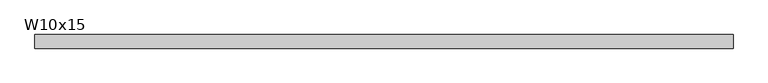
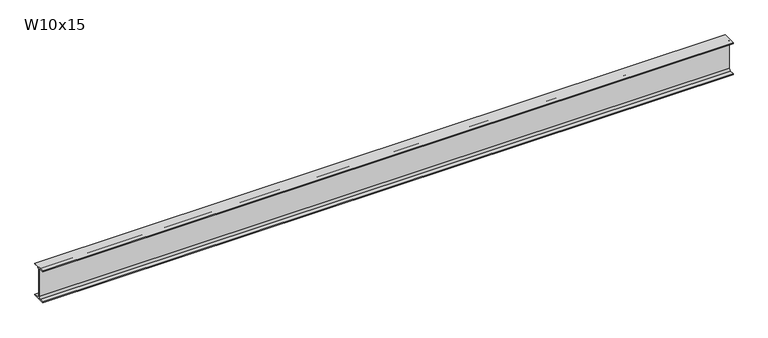
"""IFC4 building model written with IfcOpenShell, lengths in millimetres: beam geometry, RME W-Wide Flange : W10x15."""

from ifc_helpers import new_model, si_unit, point, frame, frame_2d, origin, place, context, project, spatial, polyline, circle_curve, trimmed, segment, composite_curve, outline, extrude, source, transform, mapped, element, save


def w10x15_82fe1a62(model_context):
    return source(origin(), model_context, "Body", "SweptSolid", [
        extrude(outline(composite_curve([segment(polyline([(50.8, -120.142), (50.8, -127.0), (-50.8, -127.0), (-50.8, -120.142), (-16.7005, -120.142)]), True, "CONTINUOUS"), segment(trimmed(circle_curve(frame_2d((-16.7005, -106.3625)), 13.7795), [point((-16.7005, -120.142))], [point((-2.921, -106.3625))], True, "CARTESIAN"), True, "CONTINUOUS"), segment(polyline([(-2.921, -106.3625), (-2.921, 106.3625)]), True, "CONTINUOUS"), segment(trimmed(circle_curve(frame_2d((-16.7005, 106.3625)), 13.7795), [point((-2.921, 106.3625))], [point((-16.7005, 120.142))], True, "CARTESIAN"), True, "CONTINUOUS"), segment(polyline([(-16.7005, 120.142), (-50.8, 120.142), (-50.8, 127.0), (50.8, 127.0), (50.8, 120.142), (16.7005, 120.142)]), True, "CONTINUOUS"), segment(trimmed(circle_curve(frame_2d((16.7005, 106.3625)), 13.7795), [point((16.7005, 120.142))], [point((2.921, 106.3625))], True, "CARTESIAN"), True, "CONTINUOUS"), segment(polyline([(2.921, 106.3625), (2.921, -106.3625)]), True, "CONTINUOUS"), segment(trimmed(circle_curve(frame_2d((16.7005, -106.3625)), 13.7795), [point((2.921, -106.3625))], [point((16.7005, -120.142))], True, "CARTESIAN"), True, "CONTINUOUS"), segment(polyline([(16.7005, -120.142), (50.8, -120.142)]), True, "CONTINUOUS")], self_intersect=False)), frame((-2643.5555339, 0.0, 0.0), z_axis=(1.0, 0.0, 0.0), x_axis=(0.0, 1.0, 0.0)), (0.0, 0.0, 1.0), 5197.2110143),
    ])


if __name__ == "__main__":
    model = new_model("IFC4")
    model_context = context("Model", 3, world=origin())
    ifc_project = project(units=[si_unit("LENGTHUNIT", "METRE", prefix="MILLI")], contexts=[model_context])
    site = spatial("IfcSite", under=ifc_project)
    building = spatial("IfcBuilding", under=site)
    placement = place(None, origin())
    w10x15_shape = w10x15_82fe1a62(model_context)
    element("IfcBeam", 1, ObjectType="RME W-Wide Flange : W10x15", at=placement, inside=building, context=model_context, shape_type="MappedRepresentation", body=[
        mapped(w10x15_shape, transform((0.0, 0.0, 0.0), x_axis=(1.0, 0.0, 0.0), y_axis=(0.0, 1.0, 0.0), z_axis=(0.0, 0.0, 1.0))),
    ])
    save(model, "model.ifc")

# Revit data of these elements
# Type "RME W-Wide Flange : W10x15"
#   WELD P [instance default] = ""
#   WELD LE [instance default] = ""
#   WELD D [instance default] = ""
#   TOP SECTION SIZE [instance default] = ""
#   TOP SECTION LENGTH [instance default] = ""
#   REMARKS [instance default] = ""
#   REINF TYPE [instance default] = ""
#   Nominal Size = "W24"
#   End Bearing Capacity [instance default] = ""
#   BOT SECTION SIZE [instance default] = ""
#   BOT SECTION LENGTH [instance default] = ""
#   Assembly Code = "B10"
#   W = 15
#   Start Extension Calculation [instance default] = 10' - 0"
#   Start Extension [instance default] = -0' - 0 1/2"
#   End Extension Calculation [instance default] = 10' - 0"
#   End Extension [instance default] = -0' - 0 1/2"
#   Length [instance default] = 5' - 0"
#   bf = 0' - 4"
#   d = 0' - 10"
#   k = 0' - 0 13/16"
#   k2 = 0' - 0.5425"
#   tf = 0' - 0.27"
#   tw = 0' - 0.23"
#   A = 0.030625 SF
#   Structural Material [instance default] = Metal - Steel - ASTM A992
# Element 1 (IfcBeam, "RME W-Wide Flange : W10x15")
#   Start Extension Calculation = 10' - 3.53937"
#   Start Extension = 0' - 3.03937"
#   Length = 16' - 9.07523"
#   Materials on its faces: "Metal - Steel - ASTM A992"
# Materials
#   "Metal - Steel - ASTM A992": class "Metal", colour RGB 255 128 0, transparency 0
